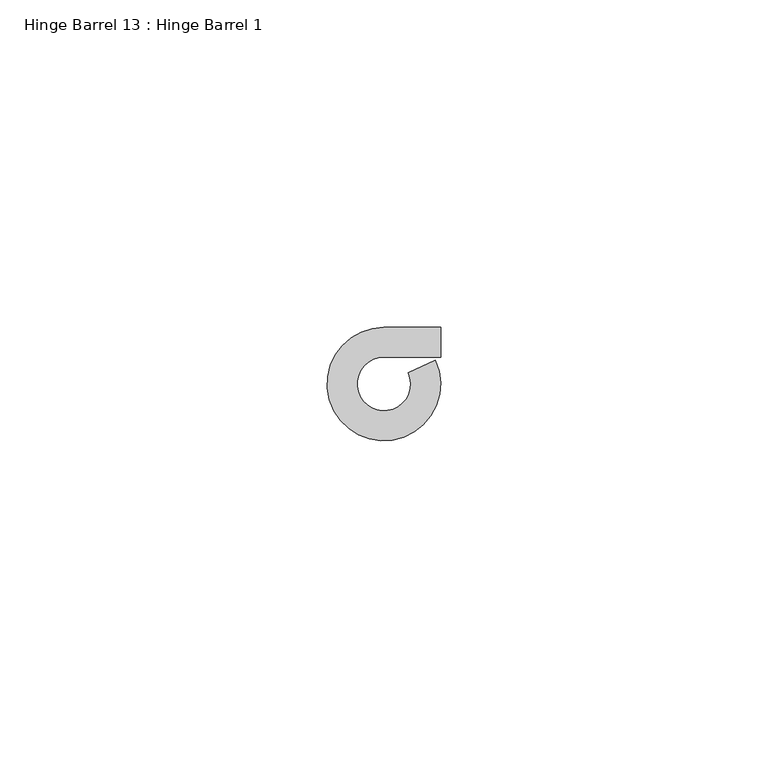
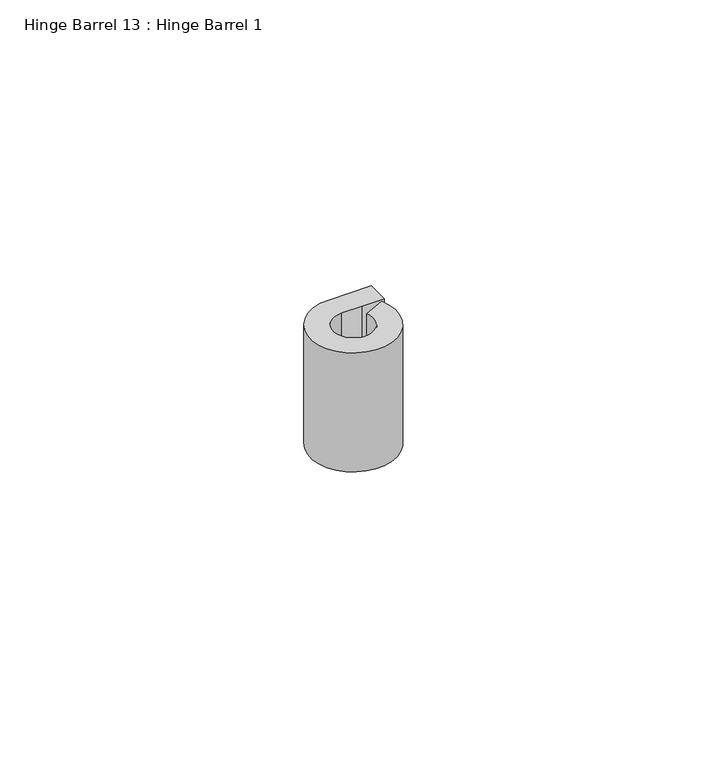
"""IFC4 building model written with IfcOpenShell, lengths in millimetres: proxy geometry, Hinge Barrel 13 : Hinge Barrel 1."""

from ifc_helpers import new_model, si_unit, point, frame, frame_2d, origin, place, context, project, spatial, polyline, circle_curve, trimmed, segment, composite_curve, outline, extrude, source, transform, mapped, element, save


def hinge_barrel_13_hinge_barrel_1_feeece1f(model_context):
    return source(origin(), model_context, "Body", "SweptSolid", [
        extrude(outline(composite_curve([segment(polyline([(587323.2214739, -533980.5883841), (587319.1320739, -533980.5883841)]), True, "CONTINUOUS"), segment(trimmed(circle_curve(frame_2d((587319.1320739, -533984.6777841)), 4.0894), [point((587319.1320739, -533980.5883841))], [point((587322.8436736, -533982.9610371))], True, "CARTESIAN"), True, "CONTINUOUS"), segment(polyline([(587322.8436736, -533982.9610371), (587326.986084, -533981.0450249)]), True, "CONTINUOUS"), segment(trimmed(circle_curve(frame_2d((587319.1320739, -533984.6777841)), 8.6534625), [point((587326.986084, -533981.0450249))], [point((587319.1320739, -533976.0243216))], False, "CARTESIAN"), True, "CONTINUOUS"), segment(polyline([(587319.1320739, -533976.0243216), (587327.7934739, -533976.0243216), (587327.7934739, -533980.5883841), (587323.2214739, -533980.5883841)]), True, "CONTINUOUS")], self_intersect=False)), frame((0.0, 0.0, 311.15), z_axis=(0.0, 0.0, 1.0), x_axis=(1.0, 0.0, 0.0)), (0.0, 0.0, 1.0), 25.4),
    ])


if __name__ == "__main__":
    model = new_model("IFC4")
    model_context = context("Model", 3, world=origin())
    ifc_project = project(units=[si_unit("LENGTHUNIT", "METRE", prefix="MILLI")], contexts=[model_context])
    site = spatial("IfcSite", under=ifc_project)
    building = spatial("IfcBuilding", under=site)
    placement = place(None, origin())
    hinge_barrel_13_hinge_barrel_1_shape = hinge_barrel_13_hinge_barrel_1_feeece1f(model_context)
    element("IfcBuildingElementProxy", 1, Name="Hinge Barrel 13 : Hinge Barrel 1", ObjectType="Hinge Barrel 13 : Hinge Barrel 1", at=placement, inside=building, context=model_context, shape_type="MappedRepresentation", body=[
        mapped(hinge_barrel_13_hinge_barrel_1_shape, transform((0.0, 0.0, 0.0), x_axis=(1.0, 0.0, 0.0), y_axis=(0.0, 1.0, 0.0), z_axis=(0.0, 0.0, 1.0))),
    ])
    save(model, "model.ifc")

# Revit data of these elements
# Element 1 (IfcBuildingElementProxy, "Hinge Barrel 13 : Hinge Barrel 1")
#   Materials on its faces: "6\"X6\" WELD-ON STL BUTT HINGE"
# Materials
#   "6\"X6\" WELD-ON STL BUTT HINGE": class "Metal", colour RGB 189 187 185, transparency 0, Description = "Carbon steel", Cost = 0
